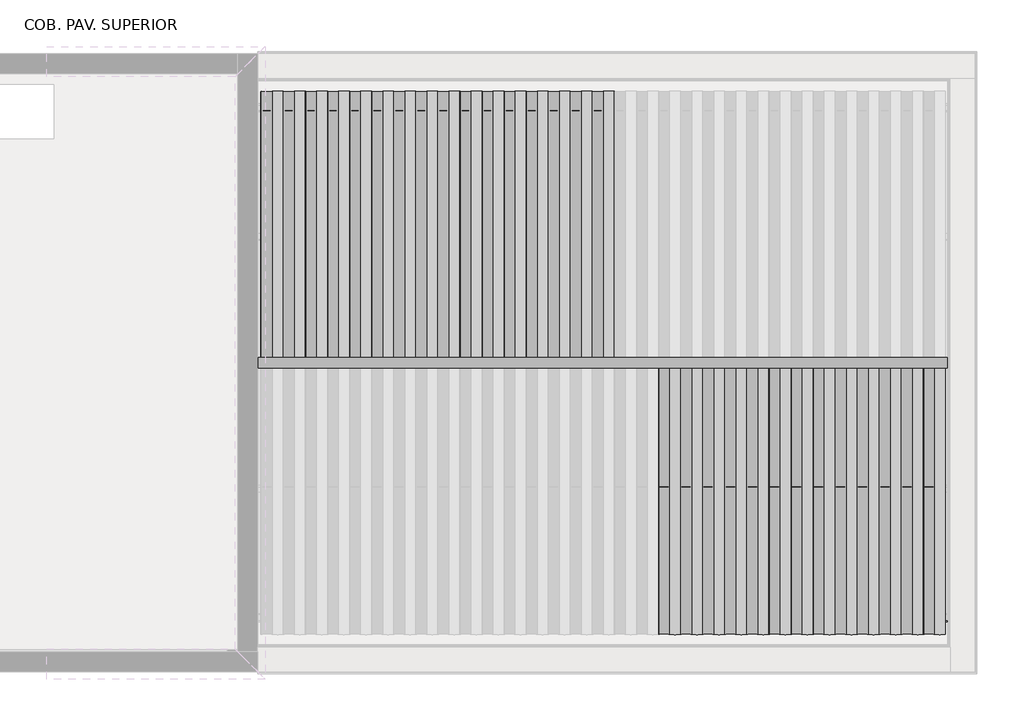
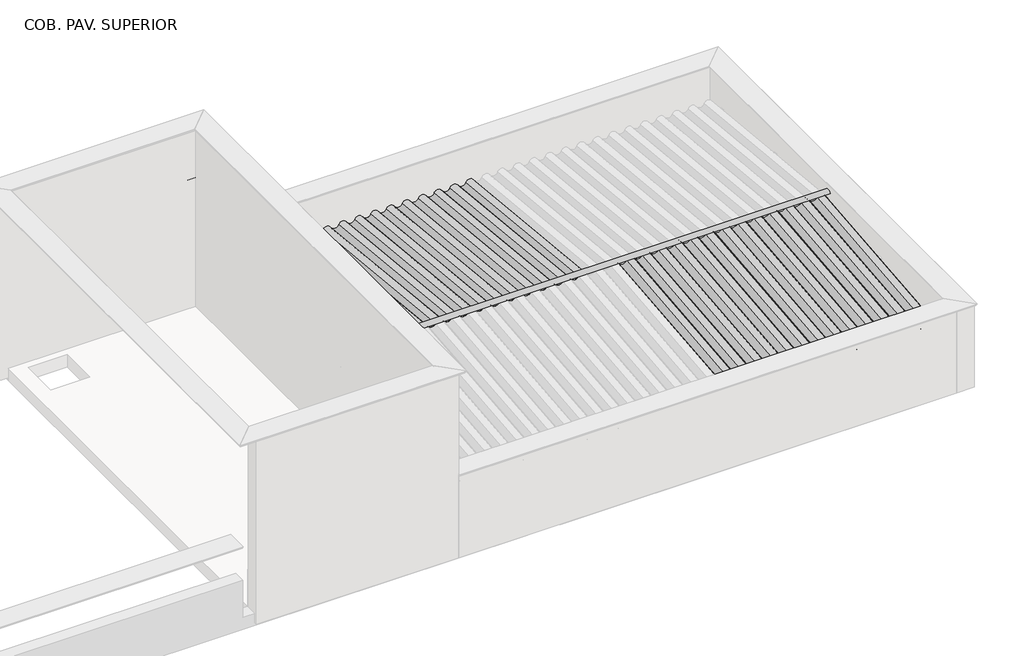
# One storey, part 6 of 7: 39 beams, 8 columns.
"""IFC4 building model written with IfcOpenShell, lengths in millimetres."""

import ifcopenshell
import ifcopenshell.guid

model = None  # the IFC model being written
_history = None  # IfcOwnerHistory: only IFC2X3 demands one
_inside = {}  # id of a spatial element -> (the spatial element, [elements in it])
_under = {}  # id of a project, library or spatial element -> (it, [spatial elements below it])
_declared = {}  # id of a project -> (the project, [libraries it declares])
_typed = {}  # id of a type object -> (the type object, [elements of that type])
_made_of = {}  # id of a material, layer set ... -> (it, [elements and type objects made of it])


def new_model(schema):
    """Start an empty IFC model of exactly this schema.

    Asked for "IFC4X3", IfcOpenShell would pick the latest addendum, in which some entities
    have other attributes; the version numbers below select the first issue.
    IFC2X3 requires an IfcOwnerHistory on every rooted entity: one is made here for all.
    """
    global model, _history
    if schema == "IFC4X3":
        model = ifcopenshell.file(schema_version=(4, 3, 0, 0))
    else:
        model = ifcopenshell.file(schema=schema)
    _inside.clear()
    _under.clear()
    _declared.clear()
    _typed.clear()
    _made_of.clear()
    _history = None
    if model.schema == "IFC2X3":
        org = make("IfcOrganization", Name="unknown")
        user = make(
            "IfcPersonAndOrganization",
            ThePerson=make("IfcPerson", FamilyName="unknown"),
            TheOrganization=org,
        )
        app = make(
            "IfcApplication",
            ApplicationDeveloper=org,
            Version="unknown",
            ApplicationFullName="unknown",
            ApplicationIdentifier="unknown",
        )
        _history = make(
            "IfcOwnerHistory",
            OwningUser=user,
            OwningApplication=app,
            ChangeAction="ADDED",
            CreationDate=0,
        )
    return model


def make(cls, **values):
    """One entity of the class cls with the attributes given. An attribute that is None is left unset."""
    return model.create_entity(
        cls, **{name: value for name, value in values.items() if value is not None}
    )


def rooted(cls, **values):
    """An entity with a GlobalId (a new one), such as an element, a storey or a relation."""
    return make(cls, GlobalId=ifcopenshell.guid.new(), OwnerHistory=_history, **values)


def si_unit(unit_type, name, prefix=None):
    """IfcSIUnit, for example si_unit("LENGTHUNIT", "METRE", prefix="MILLI")."""
    return make("IfcSIUnit", UnitType=unit_type, Prefix=prefix, Name=name)


def assignment(units):
    """IfcUnitAssignment: the units of a project."""
    return None if units is None else make("IfcUnitAssignment", Units=units)


def point(xyz):
    """IfcCartesianPoint."""
    return None if xyz is None else make("IfcCartesianPoint", Coordinates=xyz)


def direction(xyz):
    """IfcDirection."""
    return None if xyz is None else make("IfcDirection", DirectionRatios=xyz)


def frame(location, z_axis=None, x_axis=None):
    """IfcAxis2Placement3D, a coordinate frame: its origin and axes. An axis left out is left unset."""
    return make(
        "IfcAxis2Placement3D",
        Location=point(location),
        Axis=direction(z_axis),
        RefDirection=direction(x_axis),
    )


def frame_2d(location, x_axis=None):
    """IfcAxis2Placement2D, a coordinate frame in the plane: its origin and x axis."""
    return make(
        "IfcAxis2Placement2D", Location=point(location), RefDirection=direction(x_axis)
    )


def origin():
    """The frame at (0, 0, 0) with its axes left unset."""
    return frame((0.0, 0.0, 0.0))


def place(relative_to, where):
    """IfcLocalPlacement: puts the frame where relative to a parent placement (None: the world)."""
    return make(
        "IfcLocalPlacement", PlacementRelTo=relative_to, RelativePlacement=where
    )


def context(
    kind, dimensions, precision=None, world=None, true_north=None, identifier=None
):
    """IfcGeometricRepresentationContext, for example the 3D "Model" context."""
    return make(
        "IfcGeometricRepresentationContext",
        ContextIdentifier=identifier,
        ContextType=kind,
        CoordinateSpaceDimension=dimensions,
        Precision=precision,
        WorldCoordinateSystem=world,
        TrueNorth=true_north,
    )


def project(units=None, contexts=None):
    """IfcProject with its units and contexts."""
    return rooted(
        "IfcProject",
        Name="project",
        RepresentationContexts=contexts,
        UnitsInContext=assignment(units),
    )


def spatial(cls, under=None, at=None, **own):
    """A site, building, storey or space (cls), placed at a placement, below another one or the project."""
    s = rooted(cls, ObjectPlacement=at, **own)
    if under is not None:
        _under.setdefault(under.id(), (under, []))[1].append(s)
    return s


def polyline(points):
    """IfcPolyline through the points."""
    return make("IfcPolyline", Points=[point(p) for p in points])


def circle_curve(where, radius):
    """IfcCircle in the frame where."""
    return make("IfcCircle", Position=where, Radius=radius)


def trimmed(basis, trim1, trim2, sense, master):
    """IfcTrimmedCurve: the piece of a basis curve between two trims."""
    return make(
        "IfcTrimmedCurve",
        BasisCurve=basis,
        Trim1=trim1,
        Trim2=trim2,
        SenseAgreement=sense,
        MasterRepresentation=master,
    )


def segment(curve, same_sense, transition):
    """IfcCompositeCurveSegment."""
    return make(
        "IfcCompositeCurveSegment",
        Transition=transition,
        SameSense=same_sense,
        ParentCurve=curve,
    )


def composite_curve(segments, self_intersect=None):
    """IfcCompositeCurve: segments joined end to end."""
    return make("IfcCompositeCurve", Segments=segments, SelfIntersect=self_intersect)


def outline(outer, holes=None, kind="AREA"):
    """IfcArbitraryClosedProfileDef: a profile drawn as a closed curve; with holes, ...WithVoids."""
    if holes is None:
        return make("IfcArbitraryClosedProfileDef", ProfileType=kind, OuterCurve=outer)
    return make(
        "IfcArbitraryProfileDefWithVoids",
        ProfileType=kind,
        OuterCurve=outer,
        InnerCurves=holes,
    )


def extrude(swept, where, along, depth):
    """IfcExtrudedAreaSolid: the profile swept, set in the frame where, extruded along a direction by depth."""
    return make(
        "IfcExtrudedAreaSolid",
        SweptArea=swept,
        Position=where,
        ExtrudedDirection=direction(along),
        Depth=depth,
    )


def faces_of(points, faces, orient=None, outer=None):
    """IfcFace entities. A face is a list of loops; a loop is a list of indices into points, from 0.

    orient and outer hold one flag for each loop. By default every Orientation is true, the
    first loop of a face is its IfcFaceOuterBound and the others are IfcFaceBound.
    """
    made = []
    for i, loops in enumerate(faces):
        bounds = []
        for j, loop in enumerate(loops):
            is_outer = j == 0 if outer is None else outer[i][j]
            bounds.append(
                make(
                    "IfcFaceOuterBound" if is_outer else "IfcFaceBound",
                    Bound=make("IfcPolyLoop", Polygon=[points[k] for k in loop]),
                    Orientation=True if orient is None else orient[i][j],
                )
            )
        made.append(make("IfcFace", Bounds=bounds))
    return made


def faceted_brep(points, faces, orient=None, outer=None, voids=None):
    """IfcFacetedBrep: a solid bounded by flat faces; with voids (closed shells), ...WithVoids."""
    shared = [point(p) for p in points]
    hull = make("IfcClosedShell", CfsFaces=faces_of(shared, faces, orient, outer))
    if voids is None:
        return make("IfcFacetedBrep", Outer=hull)
    return make(
        "IfcFacetedBrepWithVoids",
        Outer=hull,
        Voids=[
            make(cls, CfsFaces=faces_of(shared, fs, o, b)) for cls, fs, o, b in voids
        ],
    )


def shape(context_of_items, identifier, shape_type, items):
    """IfcShapeRepresentation: the items that make up one representation, for example the "Body"."""
    return make(
        "IfcShapeRepresentation",
        ContextOfItems=context_of_items,
        RepresentationIdentifier=identifier,
        RepresentationType=shape_type,
        Items=items,
    )


def source(mapping_origin, context_of_items, identifier, shape_type, items):
    """IfcRepresentationMap: a shape defined once, which mapped items show again and again."""
    return make(
        "IfcRepresentationMap",
        MappingOrigin=mapping_origin,
        MappedRepresentation=shape(context_of_items, identifier, shape_type, items),
    )


def transform(
    local_origin,
    x_axis=None,
    y_axis=None,
    z_axis=None,
    scale=None,
    scale2=None,
    scale3=None,
    uniform=True,
):
    """IfcCartesianTransformationOperator3D, or its non-uniform kind. x_axis, y_axis, z_axis: its Axis1, 2, 3."""
    if uniform:
        return make(
            "IfcCartesianTransformationOperator3D",
            Axis1=direction(x_axis),
            Axis2=direction(y_axis),
            LocalOrigin=point(local_origin),
            Scale=scale,
            Axis3=direction(z_axis),
        )
    return make(
        "IfcCartesianTransformationOperator3DnonUniform",
        Axis1=direction(x_axis),
        Axis2=direction(y_axis),
        LocalOrigin=point(local_origin),
        Scale=scale,
        Axis3=direction(z_axis),
        Scale2=scale2,
        Scale3=scale3,
    )


def mapped(mapping_source, mapping_target):
    """IfcMappedItem: shows the shape of a source again, moved by a transform."""
    return make(
        "IfcMappedItem", MappingSource=mapping_source, MappingTarget=mapping_target
    )


def made_of(thing, what):
    """Note that an element or type object is made of a material, layer set ...; save() writes the relation."""
    if what is not None:
        _made_of.setdefault(what.id(), (what, []))[1].append(thing)
    return thing


def element(
    cls,
    number,
    at=None,
    inside=None,
    cuts=None,
    type_object=None,
    material=None,
    context=None,
    identifier="Body",
    shape_type=None,
    held_by="IfcProductDefinitionShape",
    body=None,
    shapes=None,
    **own,
):
    """One element of the class cls, such as IfcWall. Its Tag is "e" and its number.

    at: its placement. inside: the storey or other place that contains it. cuts: it is an
    opening in that element (IfcRelVoidsElement). A single representation is given by context,
    identifier, shape_type and body (its items); several are given by shapes. held_by: the class
    of the entity that holds the representations. save() writes the other relations.
    """
    e = rooted(cls, Tag="e%d" % number, ObjectPlacement=at, **own)
    if body is not None:
        shapes = [shape(context, identifier, shape_type, body)]
    if shapes is not None:
        e.Representation = make(held_by, Representations=shapes)
    if inside is not None:
        _inside.setdefault(inside.id(), (inside, []))[1].append(e)
    if cuts is not None:
        rooted(
            "IfcRelVoidsElement", RelatingBuildingElement=cuts, RelatedOpeningElement=e
        )
    if type_object is not None:
        _typed.setdefault(type_object.id(), (type_object, []))[1].append(e)
    return made_of(e, material)


def aggregate(whole, parts):
    """IfcRelAggregates: a whole, such as a stair, and the parts it consists of."""
    return rooted("IfcRelAggregates", RelatingObject=whole, RelatedObjects=parts)


def save(model, path):
    """Write the relations noted so far, then the file.

    IfcRelAggregates (storeys below a building ...), IfcRelContainedInSpatialStructure (elements
    in a storey), IfcRelDefinesByType, IfcRelAssociatesMaterial and IfcRelDeclares: one each for
    every whole, place, type object, material and project.
    """
    for whole, parts in _under.values():
        aggregate(whole, parts)
    for where, things in _inside.values():
        rooted(
            "IfcRelContainedInSpatialStructure",
            RelatedElements=things,
            RelatingStructure=where,
        )
    for kind, things in _typed.values():
        rooted("IfcRelDefinesByType", RelatedObjects=things, RelatingType=kind)
    for what, things in _made_of.values():
        rooted("IfcRelAssociatesMaterial", RelatedObjects=things, RelatingMaterial=what)
    for by, libraries in _declared.values():
        rooted("IfcRelDeclares", RelatingContext=by, RelatedDefinitions=libraries)
    model.write(path)


def cumeeira_telha_ondulada_fibrocimento_a8dbf5af(model_context):
    return source(origin(), model_context, "Body", "SweptSolid", [
        extrude(outline(composite_curve([segment(polyline([(58.3970135, 42.4437972), (53.9055884, 40.2467307)]), True, "CONTINUOUS"), segment(trimmed(circle_curve(frame_2d((-1.6029865, 13.0936483)), 61.7939461), [point((53.9055884, 40.2467307))], [point((-57.1115615, 40.2467307))], True, "CARTESIAN"), True, "CONTINUOUS"), segment(polyline([(-57.1115615, 40.2467307), (-61.6029865, 42.4437972)]), True, "CONTINUOUS"), segment(trimmed(circle_curve(frame_2d((-1.6029865, 13.0936483)), 66.7939461), [point((-61.6029865, 42.4437972))], [point((58.3970135, 42.4437972))], False, "CARTESIAN"), True, "CONTINUOUS")], self_intersect=False)), frame((-3970.0, 0.0, 0.0), z_axis=(1.0, 0.0, 0.0), x_axis=(0.0, 1.0, 0.0)), (0.0, 0.0, 1.0), 7940.0),
    ])


def viga_cumeeira_6x16cm_8fcfcc43(model_context):
    return source(origin(), model_context, "Body", "SweptSolid", [
        extrude(outline(polyline([(3822.5, 30.0), (3822.5, -30.0), (-3822.5, -30.0), (-3822.5, 30.0), (3822.5, 30.0)])), frame((0.0, 0.0, -80.0), z_axis=(0.0, 0.0, 1.0), x_axis=(1.0, 0.0, 0.0)), (0.0, 0.0, 1.0), 160.0),
    ])


def column_d505325c(model_context):
    return source(origin(), model_context, "Body", "SweptSolid", [
        extrude(outline(polyline([(30.0, 80.0), (30.0, -80.0), (-30.0, -80.0), (-30.0, 80.0), (30.0, 80.0)])), frame((0.0, 0.0, 6710.0), z_axis=(0.0, 0.0, 1.0), x_axis=(1.0, 0.0, 0.0)), (0.0, 0.0, 1.0), 750.0),
    ])


def column_4db371bd(model_context):
    return source(origin(), model_context, "Body", "SweptSolid", [
        extrude(outline(polyline([(30.0, 80.0), (30.0, -80.0), (-30.0, -80.0), (-30.0, 80.0), (30.0, 80.0)])), frame((0.0, 0.0, 6710.0), z_axis=(0.0, 0.0, 1.0), x_axis=(1.0, 0.0, 0.0)), (0.0, 0.0, 1.0), 660.0),
    ])


def column_e8b88e91(model_context):
    return source(origin(), model_context, "Body", "SweptSolid", [
        extrude(outline(polyline([(30.0, 80.0), (30.0, -80.0), (-30.0, -80.0), (-30.0, 80.0), (30.0, 80.0)])), frame((0.0, 0.0, 6710.0), z_axis=(0.0, 0.0, 1.0), x_axis=(1.0, 0.0, 0.0)), (0.0, 0.0, 1.0), 515.0),
    ])


model = new_model("IFC4")

# Units and contexts
model_context = context("Model", 3, world=origin())
ifc_project = project(units=[si_unit("LENGTHUNIT", "METRE", prefix="MILLI")], contexts=[model_context])

# Site, building, storey
site = spatial("IfcSite", under=ifc_project)
building = spatial("IfcBuilding", under=site)
storey = spatial("IfcBuildingStorey", under=building, Name="COB. PAV. SUPERIOR", Elevation=6650.0)

# Beams
placement = place(None, origin())
element("IfcBeam", 1, at=placement, inside=storey, context=model_context, shape_type="SweptSolid", body=[
    extrude(outline(polyline([(5090.718693, -7711.5607799), (5090.718693, -7831.5607799), (3090.718693, -7831.5607799), (3090.718693, -7711.5607799), (5090.718693, -7711.5607799)])), frame((0.0, 0.0, 6650.0), z_axis=(0.0, 0.0, 1.0), x_axis=(1.0, 0.0, 0.0)), (0.0, 0.0, 1.0), 60.0),
])
element("IfcBeam", 2, at=placement, inside=storey, context=model_context, shape_type="SweptSolid", body=[
    extrude(outline(polyline([(7090.718693, -7711.5607799), (7090.718693, -7831.5607799), (5090.718693, -7831.5607799), (5090.718693, -7711.5607799), (7090.718693, -7711.5607799)])), frame((0.0, 0.0, 6650.0), z_axis=(0.0, 0.0, 1.0), x_axis=(1.0, 0.0, 0.0)), (0.0, 0.0, 1.0), 60.0),
])
element("IfcBeam", 3, at=placement, inside=storey, context=model_context, shape_type="SweptSolid", body=[
    extrude(outline(polyline([(5089.7186924, -6319.8711004), (5089.7186924, -6439.8711004), (3089.718693, -6439.8711004), (3089.718693, -6319.8711004), (5089.7186924, -6319.8711004)])), frame((0.0, 0.0, 6650.0), z_axis=(0.0, 0.0, 1.0), x_axis=(1.0, 0.0, 0.0)), (0.0, 0.0, 1.0), 60.0),
])
element("IfcBeam", 4, at=placement, inside=storey, context=model_context, shape_type="SweptSolid", body=[
    extrude(outline(polyline([(7089.7186924, -6319.8711004), (7089.7186924, -6439.8711004), (5089.7186936, -6439.8711004), (5089.7186936, -6319.8711004), (7089.7186924, -6319.8711004)])), frame((0.0, 0.0, 6650.0), z_axis=(0.0, 0.0, 1.0), x_axis=(1.0, 0.0, 0.0)), (0.0, 0.0, 1.0), 60.0),
])
element("IfcBeam", 5, at=placement, inside=storey, context=model_context, shape_type="SweptSolid", body=[
    extrude(outline(polyline([(9089.718693, -9101.268869), (9089.718693, -9221.268869), (7089.718693, -9221.268869), (7089.718693, -9101.268869), (9089.718693, -9101.268869)])), frame((0.0, 0.0, 6650.0), z_axis=(0.0, 0.0, 1.0), x_axis=(1.0, 0.0, 0.0)), (0.0, 0.0, 1.0), 60.0),
])
element("IfcBeam", 6, at=placement, inside=storey, context=model_context, shape_type="SweptSolid", body=[
    extrude(outline(polyline([(9089.718693, -10521.818869), (9089.718693, -10641.818869), (7089.718693, -10641.818869), (7089.718693, -10521.818869), (9089.718693, -10521.818869)])), frame((0.0, 0.0, 6650.0), z_axis=(0.0, 0.0, 1.0), x_axis=(1.0, 0.0, 0.0)), (0.0, 0.0, 1.0), 60.0),
])
element("IfcBeam", 7, at=placement, inside=storey, context=model_context, shape_type="SweptSolid", body=[
    extrude(outline(polyline([(10709.718693, -9101.268869), (10709.718693, -9221.268869), (9089.718693, -9221.268869), (9089.718693, -9101.268869), (10709.718693, -9101.268869)])), frame((0.0, 0.0, 6650.0), z_axis=(0.0, 0.0, 1.0), x_axis=(1.0, 0.0, 0.0)), (0.0, 0.0, 1.0), 60.0),
])
element("IfcBeam", 8, at=placement, inside=storey, context=model_context, shape_type="SweptSolid", body=[
    extrude(outline(polyline([(10729.718693, -10521.818869), (10729.718693, -10641.818869), (9089.718693, -10641.818869), (9089.718693, -10521.818869), (10729.718693, -10521.818869)])), frame((0.0, 0.0, 6650.0), z_axis=(0.0, 0.0, 1.0), x_axis=(1.0, 0.0, 0.0)), (0.0, 0.0, 1.0), 60.0),
])
cumeeira_telha_ondulada_fibrocimento_shape = cumeeira_telha_ondulada_fibrocimento_a8dbf5af(model_context)
element("IfcBeam", 9, ObjectType="Cumeeira Telha Ondulada : Fibrocimento", at=placement, inside=storey, context=model_context, shape_type="MappedRepresentation", body=[
    mapped(cumeeira_telha_ondulada_fibrocimento_shape, transform((7061.718693, -7771.5607799, 7660.6251229), x_axis=(-1.0, 0.0, 0.0), y_axis=(0.0, -1.0, 0.0), z_axis=(0.0, 0.0, 1.0))),
])
element("IfcBeam", 10, ObjectType="Telha Ondulada : Fibrocimento", at=placement, inside=storey, context=model_context, shape_type="SweptSolid", body=[
    extrude(outline(composite_curve([segment(trimmed(circle_curve(frame_2d((-58.7002978, -53.2060539)), 66.7939461), [point((-29.3501489, 6.7939461))], [point((-29.3501489, -113.2060539))], False, "CARTESIAN"), True, "CONTINUOUS"), segment(polyline([(-29.3501489, -113.2060539), (-31.5472154, -108.7146289)]), True, "CONTINUOUS"), segment(trimmed(circle_curve(frame_2d((-58.7002978, -53.2060539)), 61.7939461), [point((-31.5472154, -108.7146289))], [point((-31.5472154, 2.3025211))], True, "CARTESIAN"), True, "CONTINUOUS"), segment(trimmed(circle_curve(frame_2d((0.0, 66.7939461)), 71.7939461), [point((-31.5472154, 2.3025211))], [point((-31.5472154, 131.2853711))], False, "CARTESIAN"), True, "CONTINUOUS"), segment(polyline([(-31.5472154, 131.2853711), (-29.3501489, 126.7939461)]), True, "CONTINUOUS"), segment(trimmed(circle_curve(frame_2d((0.0, 66.7939461)), 66.7939461), [point((-29.3501489, 126.7939461))], [point((-29.3501489, 6.7939461))], True, "CARTESIAN"), True, "CONTINUOUS")], self_intersect=False)), frame((3256.1156257, -4759.1621575, 7394.5315886), z_axis=(0.0, -0.9950371902099893, 0.09950371902099778), x_axis=(0.0, 0.09950371902099778, 0.9950371902099893)), (0.0, 0.0, 1.0), 3017.2387654),
])
element("IfcBeam", 11, ObjectType="Telha Ondulada : Fibrocimento", at=placement, inside=storey, context=model_context, shape_type="SweptSolid", body=[
    extrude(outline(composite_curve([segment(trimmed(circle_curve(frame_2d((-58.7002978, -53.2060539)), 66.7939461), [point((-29.3501489, 6.7939461))], [point((-29.3501489, -113.2060539))], False, "CARTESIAN"), True, "CONTINUOUS"), segment(polyline([(-29.3501489, -113.2060539), (-31.5472154, -108.7146289)]), True, "CONTINUOUS"), segment(trimmed(circle_curve(frame_2d((-58.7002978, -53.2060539)), 61.7939461), [point((-31.5472154, -108.7146289))], [point((-31.5472154, 2.3025211))], True, "CARTESIAN"), True, "CONTINUOUS"), segment(trimmed(circle_curve(frame_2d((0.0, 66.7939461)), 71.7939461), [point((-31.5472154, 2.3025211))], [point((-31.5472154, 131.2853711))], False, "CARTESIAN"), True, "CONTINUOUS"), segment(polyline([(-31.5472154, 131.2853711), (-29.3501489, 126.7939461)]), True, "CONTINUOUS"), segment(trimmed(circle_curve(frame_2d((0.0, 66.7939461)), 66.7939461), [point((-29.3501489, 126.7939461))], [point((-29.3501489, 6.7939461))], True, "CARTESIAN"), True, "CONTINUOUS")], self_intersect=False)), frame((3500.6156257, -4759.1621575, 7394.5315886), z_axis=(0.0, -0.9950371902099893, 0.09950371902099778), x_axis=(0.0, 0.09950371902099778, 0.9950371902099893)), (0.0, 0.0, 1.0), 3017.2387654),
])
element("IfcBeam", 12, ObjectType="Telha Ondulada : Fibrocimento", at=placement, inside=storey, context=model_context, shape_type="SweptSolid", body=[
    extrude(outline(composite_curve([segment(trimmed(circle_curve(frame_2d((-58.7002978, -53.2060539)), 66.7939461), [point((-29.3501489, 6.7939461))], [point((-29.3501489, -113.2060539))], False, "CARTESIAN"), True, "CONTINUOUS"), segment(polyline([(-29.3501489, -113.2060539), (-31.5472154, -108.7146289)]), True, "CONTINUOUS"), segment(trimmed(circle_curve(frame_2d((-58.7002978, -53.2060539)), 61.7939461), [point((-31.5472154, -108.7146289))], [point((-31.5472154, 2.3025211))], True, "CARTESIAN"), True, "CONTINUOUS"), segment(trimmed(circle_curve(frame_2d((0.0, 66.7939461)), 71.7939461), [point((-31.5472154, 2.3025211))], [point((-31.5472154, 131.2853711))], False, "CARTESIAN"), True, "CONTINUOUS"), segment(polyline([(-31.5472154, 131.2853711), (-29.3501489, 126.7939461)]), True, "CONTINUOUS"), segment(trimmed(circle_curve(frame_2d((0.0, 66.7939461)), 66.7939461), [point((-29.3501489, 126.7939461))], [point((-29.3501489, 6.7939461))], True, "CARTESIAN"), True, "CONTINUOUS")], self_intersect=False)), frame((3745.1156257, -4759.1621575, 7394.5315886), z_axis=(0.0, -0.9950371902099893, 0.09950371902099776), x_axis=(0.0, 0.09950371902099776, 0.9950371902099893)), (0.0, 0.0, 1.0), 3017.2387654),
])
element("IfcBeam", 13, ObjectType="Telha Ondulada : Fibrocimento", at=placement, inside=storey, context=model_context, shape_type="SweptSolid", body=[
    extrude(outline(composite_curve([segment(trimmed(circle_curve(frame_2d((-58.7002978, -53.2060539)), 66.7939461), [point((-29.3501489, 6.7939461))], [point((-29.3501489, -113.2060539))], False, "CARTESIAN"), True, "CONTINUOUS"), segment(polyline([(-29.3501489, -113.2060539), (-31.5472154, -108.7146289)]), True, "CONTINUOUS"), segment(trimmed(circle_curve(frame_2d((-58.7002978, -53.2060539)), 61.7939461), [point((-31.5472154, -108.7146289))], [point((-31.5472154, 2.3025211))], True, "CARTESIAN"), True, "CONTINUOUS"), segment(trimmed(circle_curve(frame_2d((0.0, 66.7939461)), 71.7939461), [point((-31.5472154, 2.3025211))], [point((-31.5472154, 131.2853711))], False, "CARTESIAN"), True, "CONTINUOUS"), segment(polyline([(-31.5472154, 131.2853711), (-29.3501489, 126.7939461)]), True, "CONTINUOUS"), segment(trimmed(circle_curve(frame_2d((0.0, 66.7939461)), 66.7939461), [point((-29.3501489, 126.7939461))], [point((-29.3501489, 6.7939461))], True, "CARTESIAN"), True, "CONTINUOUS")], self_intersect=False)), frame((3989.6156257, -4759.1621575, 7394.5315886), z_axis=(0.0, -0.9950371902099893, 0.09950371902099776), x_axis=(0.0, 0.09950371902099776, 0.9950371902099893)), (0.0, 0.0, 1.0), 3017.2387654),
])
element("IfcBeam", 14, ObjectType="Telha Ondulada : Fibrocimento", at=placement, inside=storey, context=model_context, shape_type="SweptSolid", body=[
    extrude(outline(composite_curve([segment(trimmed(circle_curve(frame_2d((-58.7002978, -53.2060539)), 66.7939461), [point((-29.3501489, 6.7939461))], [point((-29.3501489, -113.2060539))], False, "CARTESIAN"), True, "CONTINUOUS"), segment(polyline([(-29.3501489, -113.2060539), (-31.5472154, -108.7146289)]), True, "CONTINUOUS"), segment(trimmed(circle_curve(frame_2d((-58.7002978, -53.2060539)), 61.7939461), [point((-31.5472154, -108.7146289))], [point((-31.5472154, 2.3025211))], True, "CARTESIAN"), True, "CONTINUOUS"), segment(trimmed(circle_curve(frame_2d((0.0, 66.7939461)), 71.7939461), [point((-31.5472154, 2.3025211))], [point((-31.5472154, 131.2853711))], False, "CARTESIAN"), True, "CONTINUOUS"), segment(polyline([(-31.5472154, 131.2853711), (-29.3501489, 126.7939461)]), True, "CONTINUOUS"), segment(trimmed(circle_curve(frame_2d((0.0, 66.7939461)), 66.7939461), [point((-29.3501489, 126.7939461))], [point((-29.3501489, 6.7939461))], True, "CARTESIAN"), True, "CONTINUOUS")], self_intersect=False)), frame((4234.1156257, -4759.1621575, 7394.5315886), z_axis=(0.0, -0.9950371902099893, 0.09950371902099775), x_axis=(0.0, 0.09950371902099775, 0.9950371902099893)), (0.0, 0.0, 1.0), 3017.2387654),
])
element("IfcBeam", 15, ObjectType="Telha Ondulada : Fibrocimento", at=placement, inside=storey, context=model_context, shape_type="SweptSolid", body=[
    extrude(outline(composite_curve([segment(trimmed(circle_curve(frame_2d((-58.7002978, -53.2060539)), 66.7939461), [point((-29.3501489, 6.7939461))], [point((-29.3501489, -113.2060539))], False, "CARTESIAN"), True, "CONTINUOUS"), segment(polyline([(-29.3501489, -113.2060539), (-31.5472154, -108.7146289)]), True, "CONTINUOUS"), segment(trimmed(circle_curve(frame_2d((-58.7002978, -53.2060539)), 61.7939461), [point((-31.5472154, -108.7146289))], [point((-31.5472154, 2.3025211))], True, "CARTESIAN"), True, "CONTINUOUS"), segment(trimmed(circle_curve(frame_2d((0.0, 66.7939461)), 71.7939461), [point((-31.5472154, 2.3025211))], [point((-31.5472154, 131.2853711))], False, "CARTESIAN"), True, "CONTINUOUS"), segment(polyline([(-31.5472154, 131.2853711), (-29.3501489, 126.7939461)]), True, "CONTINUOUS"), segment(trimmed(circle_curve(frame_2d((0.0, 66.7939461)), 66.7939461), [point((-29.3501489, 126.7939461))], [point((-29.3501489, 6.7939461))], True, "CARTESIAN"), True, "CONTINUOUS")], self_intersect=False)), frame((4478.6156257, -4759.1621575, 7394.5315886), z_axis=(0.0, -0.9950371902099893, 0.09950371902099778), x_axis=(0.0, 0.09950371902099778, 0.9950371902099893)), (0.0, 0.0, 1.0), 3017.2387654),
])
element("IfcBeam", 16, ObjectType="Telha Ondulada : Fibrocimento", at=placement, inside=storey, context=model_context, shape_type="SweptSolid", body=[
    extrude(outline(composite_curve([segment(trimmed(circle_curve(frame_2d((-58.7002978, -53.2060539)), 66.7939461), [point((-29.3501489, 6.7939461))], [point((-29.3501489, -113.2060539))], False, "CARTESIAN"), True, "CONTINUOUS"), segment(polyline([(-29.3501489, -113.2060539), (-31.5472154, -108.7146289)]), True, "CONTINUOUS"), segment(trimmed(circle_curve(frame_2d((-58.7002978, -53.2060539)), 61.7939461), [point((-31.5472154, -108.7146289))], [point((-31.5472154, 2.3025211))], True, "CARTESIAN"), True, "CONTINUOUS"), segment(trimmed(circle_curve(frame_2d((0.0, 66.7939461)), 71.7939461), [point((-31.5472154, 2.3025211))], [point((-31.5472154, 131.2853711))], False, "CARTESIAN"), True, "CONTINUOUS"), segment(polyline([(-31.5472154, 131.2853711), (-29.3501489, 126.7939461)]), True, "CONTINUOUS"), segment(trimmed(circle_curve(frame_2d((0.0, 66.7939461)), 66.7939461), [point((-29.3501489, 126.7939461))], [point((-29.3501489, 6.7939461))], True, "CARTESIAN"), True, "CONTINUOUS")], self_intersect=False)), frame((4723.1156257, -4759.1621575, 7394.5315886), z_axis=(0.0, -0.9950371902099893, 0.09950371902099776), x_axis=(0.0, 0.09950371902099776, 0.9950371902099893)), (0.0, 0.0, 1.0), 3017.2387654),
])
element("IfcBeam", 17, ObjectType="Telha Ondulada : Fibrocimento", at=placement, inside=storey, context=model_context, shape_type="SweptSolid", body=[
    extrude(outline(composite_curve([segment(trimmed(circle_curve(frame_2d((-58.7002978, -53.2060539)), 66.7939461), [point((-29.3501489, 6.7939461))], [point((-29.3501489, -113.2060539))], False, "CARTESIAN"), True, "CONTINUOUS"), segment(polyline([(-29.3501489, -113.2060539), (-31.5472154, -108.7146289)]), True, "CONTINUOUS"), segment(trimmed(circle_curve(frame_2d((-58.7002978, -53.2060539)), 61.7939461), [point((-31.5472154, -108.7146289))], [point((-31.5472154, 2.3025211))], True, "CARTESIAN"), True, "CONTINUOUS"), segment(trimmed(circle_curve(frame_2d((0.0, 66.7939461)), 71.7939461), [point((-31.5472154, 2.3025211))], [point((-31.5472154, 131.2853711))], False, "CARTESIAN"), True, "CONTINUOUS"), segment(polyline([(-31.5472154, 131.2853711), (-29.3501489, 126.7939461)]), True, "CONTINUOUS"), segment(trimmed(circle_curve(frame_2d((0.0, 66.7939461)), 66.7939461), [point((-29.3501489, 126.7939461))], [point((-29.3501489, 6.7939461))], True, "CARTESIAN"), True, "CONTINUOUS")], self_intersect=False)), frame((4967.6156257, -4759.1621575, 7394.5315886), z_axis=(0.0, -0.9950371902099893, 0.09950371902099775), x_axis=(0.0, 0.09950371902099775, 0.9950371902099893)), (0.0, 0.0, 1.0), 3017.2387654),
])
element("IfcBeam", 18, ObjectType="Telha Ondulada : Fibrocimento", at=placement, inside=storey, context=model_context, shape_type="SweptSolid", body=[
    extrude(outline(composite_curve([segment(trimmed(circle_curve(frame_2d((-58.7002978, -53.2060539)), 66.7939461), [point((-29.3501489, 6.7939461))], [point((-29.3501489, -113.2060539))], False, "CARTESIAN"), True, "CONTINUOUS"), segment(polyline([(-29.3501489, -113.2060539), (-31.5472154, -108.7146289)]), True, "CONTINUOUS"), segment(trimmed(circle_curve(frame_2d((-58.7002978, -53.2060539)), 61.7939461), [point((-31.5472154, -108.7146289))], [point((-31.5472154, 2.3025211))], True, "CARTESIAN"), True, "CONTINUOUS"), segment(trimmed(circle_curve(frame_2d((0.0, 66.7939461)), 71.7939461), [point((-31.5472154, 2.3025211))], [point((-31.5472154, 131.2853711))], False, "CARTESIAN"), True, "CONTINUOUS"), segment(polyline([(-31.5472154, 131.2853711), (-29.3501489, 126.7939461)]), True, "CONTINUOUS"), segment(trimmed(circle_curve(frame_2d((0.0, 66.7939461)), 66.7939461), [point((-29.3501489, 126.7939461))], [point((-29.3501489, 6.7939461))], True, "CARTESIAN"), True, "CONTINUOUS")], self_intersect=False)), frame((5212.1156257, -4759.1621575, 7394.5315886), z_axis=(0.0, -0.9950371902099893, 0.09950371902099778), x_axis=(0.0, 0.09950371902099778, 0.9950371902099893)), (0.0, 0.0, 1.0), 3017.2387654),
])
element("IfcBeam", 19, ObjectType="Telha Ondulada : Fibrocimento", at=placement, inside=storey, context=model_context, shape_type="SweptSolid", body=[
    extrude(outline(composite_curve([segment(trimmed(circle_curve(frame_2d((-58.7002978, -53.2060539)), 66.7939461), [point((-29.3501489, 6.7939461))], [point((-29.3501489, -113.2060539))], False, "CARTESIAN"), True, "CONTINUOUS"), segment(polyline([(-29.3501489, -113.2060539), (-31.5472154, -108.7146289)]), True, "CONTINUOUS"), segment(trimmed(circle_curve(frame_2d((-58.7002978, -53.2060539)), 61.7939461), [point((-31.5472154, -108.7146289))], [point((-31.5472154, 2.3025211))], True, "CARTESIAN"), True, "CONTINUOUS"), segment(trimmed(circle_curve(frame_2d((0.0, 66.7939461)), 71.7939461), [point((-31.5472154, 2.3025211))], [point((-31.5472154, 131.2853711))], False, "CARTESIAN"), True, "CONTINUOUS"), segment(polyline([(-31.5472154, 131.2853711), (-29.3501489, 126.7939461)]), True, "CONTINUOUS"), segment(trimmed(circle_curve(frame_2d((0.0, 66.7939461)), 66.7939461), [point((-29.3501489, 126.7939461))], [point((-29.3501489, 6.7939461))], True, "CARTESIAN"), True, "CONTINUOUS")], self_intersect=False)), frame((5456.6156257, -4759.1621575, 7394.5315886), z_axis=(0.0, -0.9950371902099893, 0.09950371902099776), x_axis=(0.0, 0.09950371902099776, 0.9950371902099893)), (0.0, 0.0, 1.0), 3017.2387654),
])
element("IfcBeam", 20, ObjectType="Telha Ondulada : Fibrocimento", at=placement, inside=storey, context=model_context, shape_type="SweptSolid", body=[
    extrude(outline(composite_curve([segment(trimmed(circle_curve(frame_2d((-58.7002978, -53.2060539)), 66.7939461), [point((-29.3501489, 6.7939461))], [point((-29.3501489, -113.2060539))], False, "CARTESIAN"), True, "CONTINUOUS"), segment(polyline([(-29.3501489, -113.2060539), (-31.5472154, -108.7146289)]), True, "CONTINUOUS"), segment(trimmed(circle_curve(frame_2d((-58.7002978, -53.2060539)), 61.7939461), [point((-31.5472154, -108.7146289))], [point((-31.5472154, 2.3025211))], True, "CARTESIAN"), True, "CONTINUOUS"), segment(trimmed(circle_curve(frame_2d((0.0, 66.7939461)), 71.7939461), [point((-31.5472154, 2.3025211))], [point((-31.5472154, 131.2853711))], False, "CARTESIAN"), True, "CONTINUOUS"), segment(polyline([(-31.5472154, 131.2853711), (-29.3501489, 126.7939461)]), True, "CONTINUOUS"), segment(trimmed(circle_curve(frame_2d((0.0, 66.7939461)), 66.7939461), [point((-29.3501489, 126.7939461))], [point((-29.3501489, 6.7939461))], True, "CARTESIAN"), True, "CONTINUOUS")], self_intersect=False)), frame((5701.1156257, -4759.1621575, 7394.5315886), z_axis=(0.0, -0.9950371902099893, 0.09950371902099776), x_axis=(0.0, 0.09950371902099776, 0.9950371902099893)), (0.0, 0.0, 1.0), 3017.2387654),
])
element("IfcBeam", 21, ObjectType="Telha Ondulada : Fibrocimento", at=placement, inside=storey, context=model_context, shape_type="SweptSolid", body=[
    extrude(outline(composite_curve([segment(trimmed(circle_curve(frame_2d((-58.7002978, -53.2060539)), 66.7939461), [point((-29.3501489, 6.7939461))], [point((-29.3501489, -113.2060539))], False, "CARTESIAN"), True, "CONTINUOUS"), segment(polyline([(-29.3501489, -113.2060539), (-31.5472154, -108.7146289)]), True, "CONTINUOUS"), segment(trimmed(circle_curve(frame_2d((-58.7002978, -53.2060539)), 61.7939461), [point((-31.5472154, -108.7146289))], [point((-31.5472154, 2.3025211))], True, "CARTESIAN"), True, "CONTINUOUS"), segment(trimmed(circle_curve(frame_2d((0.0, 66.7939461)), 71.7939461), [point((-31.5472154, 2.3025211))], [point((-31.5472154, 131.2853711))], False, "CARTESIAN"), True, "CONTINUOUS"), segment(polyline([(-31.5472154, 131.2853711), (-29.3501489, 126.7939461)]), True, "CONTINUOUS"), segment(trimmed(circle_curve(frame_2d((0.0, 66.7939461)), 66.7939461), [point((-29.3501489, 126.7939461))], [point((-29.3501489, 6.7939461))], True, "CARTESIAN"), True, "CONTINUOUS")], self_intersect=False)), frame((5945.6156257, -4759.1621575, 7394.5315886), z_axis=(0.0, -0.9950371902099893, 0.09950371902099778), x_axis=(0.0, 0.09950371902099778, 0.9950371902099893)), (0.0, 0.0, 1.0), 3017.2387654),
])
element("IfcBeam", 22, ObjectType="Telha Ondulada : Fibrocimento", at=placement, inside=storey, context=model_context, shape_type="SweptSolid", body=[
    extrude(outline(composite_curve([segment(trimmed(circle_curve(frame_2d((-58.7002978, -53.2060539)), 66.7939461), [point((-29.3501489, 6.7939461))], [point((-29.3501489, -113.2060539))], False, "CARTESIAN"), True, "CONTINUOUS"), segment(polyline([(-29.3501489, -113.2060539), (-31.5472154, -108.7146289)]), True, "CONTINUOUS"), segment(trimmed(circle_curve(frame_2d((-58.7002978, -53.2060539)), 61.7939461), [point((-31.5472154, -108.7146289))], [point((-31.5472154, 2.3025211))], True, "CARTESIAN"), True, "CONTINUOUS"), segment(trimmed(circle_curve(frame_2d((0.0, 66.7939461)), 71.7939461), [point((-31.5472154, 2.3025211))], [point((-31.5472154, 131.2853711))], False, "CARTESIAN"), True, "CONTINUOUS"), segment(polyline([(-31.5472154, 131.2853711), (-29.3501489, 126.7939461)]), True, "CONTINUOUS"), segment(trimmed(circle_curve(frame_2d((0.0, 66.7939461)), 66.7939461), [point((-29.3501489, 126.7939461))], [point((-29.3501489, 6.7939461))], True, "CARTESIAN"), True, "CONTINUOUS")], self_intersect=False)), frame((6190.1156257, -4759.1621575, 7394.5315886), z_axis=(0.0, -0.9950371902099893, 0.09950371902099778), x_axis=(0.0, 0.09950371902099778, 0.9950371902099893)), (0.0, 0.0, 1.0), 3017.2387654),
])
element("IfcBeam", 23, ObjectType="Telha Ondulada : Fibrocimento", at=placement, inside=storey, context=model_context, shape_type="SweptSolid", body=[
    extrude(outline(composite_curve([segment(trimmed(circle_curve(frame_2d((-58.7002978, -53.2060539)), 66.7939461), [point((-29.3501489, 6.7939461))], [point((-29.3501489, -113.2060539))], False, "CARTESIAN"), True, "CONTINUOUS"), segment(polyline([(-29.3501489, -113.2060539), (-31.5472154, -108.7146289)]), True, "CONTINUOUS"), segment(trimmed(circle_curve(frame_2d((-58.7002978, -53.2060539)), 61.7939461), [point((-31.5472154, -108.7146289))], [point((-31.5472154, 2.3025211))], True, "CARTESIAN"), True, "CONTINUOUS"), segment(trimmed(circle_curve(frame_2d((0.0, 66.7939461)), 71.7939461), [point((-31.5472154, 2.3025211))], [point((-31.5472154, 131.2853711))], False, "CARTESIAN"), True, "CONTINUOUS"), segment(polyline([(-31.5472154, 131.2853711), (-29.3501489, 126.7939461)]), True, "CONTINUOUS"), segment(trimmed(circle_curve(frame_2d((0.0, 66.7939461)), 66.7939461), [point((-29.3501489, 126.7939461))], [point((-29.3501489, 6.7939461))], True, "CARTESIAN"), True, "CONTINUOUS")], self_intersect=False)), frame((6434.6156257, -4759.1621575, 7394.5315886), z_axis=(0.0, -0.9950371902099893, 0.09950371902099776), x_axis=(0.0, 0.09950371902099776, 0.9950371902099893)), (0.0, 0.0, 1.0), 3017.2387654),
])
element("IfcBeam", 24, ObjectType="Telha Ondulada : Fibrocimento", at=placement, inside=storey, context=model_context, shape_type="SweptSolid", body=[
    extrude(outline(composite_curve([segment(trimmed(circle_curve(frame_2d((-58.7002978, -53.2060539)), 66.7939461), [point((-29.3501489, 6.7939461))], [point((-29.3501489, -113.2060539))], False, "CARTESIAN"), True, "CONTINUOUS"), segment(polyline([(-29.3501489, -113.2060539), (-31.5472154, -108.7146289)]), True, "CONTINUOUS"), segment(trimmed(circle_curve(frame_2d((-58.7002978, -53.2060539)), 61.7939461), [point((-31.5472154, -108.7146289))], [point((-31.5472154, 2.3025211))], True, "CARTESIAN"), True, "CONTINUOUS"), segment(trimmed(circle_curve(frame_2d((0.0, 66.7939461)), 71.7939461), [point((-31.5472154, 2.3025211))], [point((-31.5472154, 131.2853711))], False, "CARTESIAN"), True, "CONTINUOUS"), segment(polyline([(-31.5472154, 131.2853711), (-29.3501489, 126.7939461)]), True, "CONTINUOUS"), segment(trimmed(circle_curve(frame_2d((0.0, 66.7939461)), 66.7939461), [point((-29.3501489, 126.7939461))], [point((-29.3501489, 6.7939461))], True, "CARTESIAN"), True, "CONTINUOUS")], self_intersect=False)), frame((6679.1156257, -4759.1621575, 7394.5315886), z_axis=(0.0, -0.9950371902099893, 0.09950371902099776), x_axis=(0.0, 0.09950371902099776, 0.9950371902099893)), (0.0, 0.0, 1.0), 3017.2387654),
])
element("IfcBeam", 25, ObjectType="Telha Ondulada : Fibrocimento", at=placement, inside=storey, context=model_context, shape_type="SweptSolid", body=[
    extrude(outline(composite_curve([segment(trimmed(circle_curve(frame_2d((-58.7002978, -53.2060539)), 66.7939461), [point((-29.3501489, 6.7939461))], [point((-29.3501489, -113.2060539))], False, "CARTESIAN"), True, "CONTINUOUS"), segment(polyline([(-29.3501489, -113.2060539), (-31.5472154, -108.7146289)]), True, "CONTINUOUS"), segment(trimmed(circle_curve(frame_2d((-58.7002978, -53.2060539)), 61.7939461), [point((-31.5472154, -108.7146289))], [point((-31.5472154, 2.3025211))], True, "CARTESIAN"), True, "CONTINUOUS"), segment(trimmed(circle_curve(frame_2d((0.0, 66.7939461)), 71.7939461), [point((-31.5472154, 2.3025211))], [point((-31.5472154, 131.2853711))], False, "CARTESIAN"), True, "CONTINUOUS"), segment(polyline([(-31.5472154, 131.2853711), (-29.3501489, 126.7939461)]), True, "CONTINUOUS"), segment(trimmed(circle_curve(frame_2d((0.0, 66.7939461)), 66.7939461), [point((-29.3501489, 126.7939461))], [point((-29.3501489, 6.7939461))], True, "CARTESIAN"), True, "CONTINUOUS")], self_intersect=False)), frame((6923.6156257, -4759.1621575, 7394.5315886), z_axis=(0.0, -0.9950371902099893, 0.09950371902099775), x_axis=(0.0, 0.09950371902099775, 0.9950371902099893)), (0.0, 0.0, 1.0), 3017.2387654),
])
element("IfcBeam", 26, ObjectType="Telha Ondulada : Fibrocimento", at=placement, inside=storey, context=model_context, shape_type="SweptSolid", body=[
    extrude(outline(composite_curve([segment(trimmed(circle_curve(frame_2d((0.0, 66.7939461)), 66.7939461), [point((29.3501489, 6.7939461))], [point((29.3501489, 126.7939461))], True, "CARTESIAN"), True, "CONTINUOUS"), segment(polyline([(29.3501489, 126.7939461), (31.5472154, 131.2853711)]), True, "CONTINUOUS"), segment(trimmed(circle_curve(frame_2d((0.0, 66.7939461)), 71.7939461), [point((31.5472154, 131.2853711))], [point((31.5472154, 2.3025211))], False, "CARTESIAN"), True, "CONTINUOUS"), segment(trimmed(circle_curve(frame_2d((58.7002978, -53.2060539)), 61.7939461), [point((31.5472154, 2.3025211))], [point((31.5472154, -108.7146289))], True, "CARTESIAN"), True, "CONTINUOUS"), segment(polyline([(31.5472154, -108.7146289), (29.3501489, -113.2060539)]), True, "CONTINUOUS"), segment(trimmed(circle_curve(frame_2d((58.7002978, -53.2060539)), 66.7939461), [point((29.3501489, -113.2060539))], [point((29.3501489, 6.7939461))], False, "CARTESIAN"), True, "CONTINUOUS")], self_intersect=False)), frame((7657.1156257, -10781.9594023, 7394.5315886), z_axis=(0.0, 0.9950371902099894, 0.09950371902099747), x_axis=(0.0, 0.09950371902099747, -0.9950371902099894)), (0.0, 0.0, 1.0), 3017.2387654),
])
element("IfcBeam", 27, ObjectType="Telha Ondulada : Fibrocimento", at=placement, inside=storey, context=model_context, shape_type="SweptSolid", body=[
    extrude(outline(composite_curve([segment(trimmed(circle_curve(frame_2d((0.0, 66.7939461)), 66.7939461), [point((29.3501489, 6.7939461))], [point((29.3501489, 126.7939461))], True, "CARTESIAN"), True, "CONTINUOUS"), segment(polyline([(29.3501489, 126.7939461), (31.5472154, 131.2853711)]), True, "CONTINUOUS"), segment(trimmed(circle_curve(frame_2d((0.0, 66.7939461)), 71.7939461), [point((31.5472154, 131.2853711))], [point((31.5472154, 2.3025211))], False, "CARTESIAN"), True, "CONTINUOUS"), segment(trimmed(circle_curve(frame_2d((58.7002978, -53.2060539)), 61.7939461), [point((31.5472154, 2.3025211))], [point((31.5472154, -108.7146289))], True, "CARTESIAN"), True, "CONTINUOUS"), segment(polyline([(31.5472154, -108.7146289), (29.3501489, -113.2060539)]), True, "CONTINUOUS"), segment(trimmed(circle_curve(frame_2d((58.7002978, -53.2060539)), 66.7939461), [point((29.3501489, -113.2060539))], [point((29.3501489, 6.7939461))], False, "CARTESIAN"), True, "CONTINUOUS")], self_intersect=False)), frame((7901.6156257, -10781.9594023, 7394.5315886), z_axis=(0.0, 0.9950371902099894, 0.09950371902099751), x_axis=(0.0, 0.09950371902099751, -0.9950371902099894)), (0.0, 0.0, 1.0), 3017.2387654),
])
element("IfcBeam", 28, ObjectType="Telha Ondulada : Fibrocimento", at=placement, inside=storey, context=model_context, shape_type="SweptSolid", body=[
    extrude(outline(composite_curve([segment(trimmed(circle_curve(frame_2d((0.0, 66.7939461)), 66.7939461), [point((29.3501489, 6.7939461))], [point((29.3501489, 126.7939461))], True, "CARTESIAN"), True, "CONTINUOUS"), segment(polyline([(29.3501489, 126.7939461), (31.5472154, 131.2853711)]), True, "CONTINUOUS"), segment(trimmed(circle_curve(frame_2d((0.0, 66.7939461)), 71.7939461), [point((31.5472154, 131.2853711))], [point((31.5472154, 2.3025211))], False, "CARTESIAN"), True, "CONTINUOUS"), segment(trimmed(circle_curve(frame_2d((58.7002978, -53.2060539)), 61.7939461), [point((31.5472154, 2.3025211))], [point((31.5472154, -108.7146289))], True, "CARTESIAN"), True, "CONTINUOUS"), segment(polyline([(31.5472154, -108.7146289), (29.3501489, -113.2060539)]), True, "CONTINUOUS"), segment(trimmed(circle_curve(frame_2d((58.7002978, -53.2060539)), 66.7939461), [point((29.3501489, -113.2060539))], [point((29.3501489, 6.7939461))], False, "CARTESIAN"), True, "CONTINUOUS")], self_intersect=False)), frame((8146.1156257, -10781.9594023, 7394.5315886), z_axis=(0.0, 0.9950371902099894, 0.09950371902099751), x_axis=(0.0, 0.09950371902099751, -0.9950371902099894)), (0.0, 0.0, 1.0), 3017.2387654),
])
element("IfcBeam", 29, ObjectType="Telha Ondulada : Fibrocimento", at=placement, inside=storey, context=model_context, shape_type="SweptSolid", body=[
    extrude(outline(composite_curve([segment(trimmed(circle_curve(frame_2d((0.0, 66.7939461)), 66.7939461), [point((29.3501489, 6.7939461))], [point((29.3501489, 126.7939461))], True, "CARTESIAN"), True, "CONTINUOUS"), segment(polyline([(29.3501489, 126.7939461), (31.5472154, 131.2853711)]), True, "CONTINUOUS"), segment(trimmed(circle_curve(frame_2d((0.0, 66.7939461)), 71.7939461), [point((31.5472154, 131.2853711))], [point((31.5472154, 2.3025211))], False, "CARTESIAN"), True, "CONTINUOUS"), segment(trimmed(circle_curve(frame_2d((58.7002978, -53.2060539)), 61.7939461), [point((31.5472154, 2.3025211))], [point((31.5472154, -108.7146289))], True, "CARTESIAN"), True, "CONTINUOUS"), segment(polyline([(31.5472154, -108.7146289), (29.3501489, -113.2060539)]), True, "CONTINUOUS"), segment(trimmed(circle_curve(frame_2d((58.7002978, -53.2060539)), 66.7939461), [point((29.3501489, -113.2060539))], [point((29.3501489, 6.7939461))], False, "CARTESIAN"), True, "CONTINUOUS")], self_intersect=False)), frame((8390.6156257, -10781.9594023, 7394.5315886), z_axis=(0.0, 0.9950371902099894, 0.09950371902099751), x_axis=(0.0, 0.09950371902099751, -0.9950371902099894)), (0.0, 0.0, 1.0), 3017.2387654),
])
element("IfcBeam", 30, ObjectType="Telha Ondulada : Fibrocimento", at=placement, inside=storey, context=model_context, shape_type="SweptSolid", body=[
    extrude(outline(composite_curve([segment(trimmed(circle_curve(frame_2d((0.0, 66.7939461)), 66.7939461), [point((29.3501489, 6.7939461))], [point((29.3501489, 126.7939461))], True, "CARTESIAN"), True, "CONTINUOUS"), segment(polyline([(29.3501489, 126.7939461), (31.5472154, 131.2853711)]), True, "CONTINUOUS"), segment(trimmed(circle_curve(frame_2d((0.0, 66.7939461)), 71.7939461), [point((31.5472154, 131.2853711))], [point((31.5472154, 2.3025211))], False, "CARTESIAN"), True, "CONTINUOUS"), segment(trimmed(circle_curve(frame_2d((58.7002978, -53.2060539)), 61.7939461), [point((31.5472154, 2.3025211))], [point((31.5472154, -108.7146289))], True, "CARTESIAN"), True, "CONTINUOUS"), segment(polyline([(31.5472154, -108.7146289), (29.3501489, -113.2060539)]), True, "CONTINUOUS"), segment(trimmed(circle_curve(frame_2d((58.7002978, -53.2060539)), 66.7939461), [point((29.3501489, -113.2060539))], [point((29.3501489, 6.7939461))], False, "CARTESIAN"), True, "CONTINUOUS")], self_intersect=False)), frame((8635.1156257, -10781.9594023, 7394.5315886), z_axis=(0.0, 0.9950371902099894, 0.09950371902099747), x_axis=(0.0, 0.09950371902099747, -0.9950371902099894)), (0.0, 0.0, 1.0), 3017.2387654),
])
element("IfcBeam", 31, ObjectType="Telha Ondulada : Fibrocimento", at=placement, inside=storey, context=model_context, shape_type="SweptSolid", body=[
    extrude(outline(composite_curve([segment(trimmed(circle_curve(frame_2d((0.0, 66.7939461)), 66.7939461), [point((29.3501489, 6.7939461))], [point((29.3501489, 126.7939461))], True, "CARTESIAN"), True, "CONTINUOUS"), segment(polyline([(29.3501489, 126.7939461), (31.5472154, 131.2853711)]), True, "CONTINUOUS"), segment(trimmed(circle_curve(frame_2d((0.0, 66.7939461)), 71.7939461), [point((31.5472154, 131.2853711))], [point((31.5472154, 2.3025211))], False, "CARTESIAN"), True, "CONTINUOUS"), segment(trimmed(circle_curve(frame_2d((58.7002978, -53.2060539)), 61.7939461), [point((31.5472154, 2.3025211))], [point((31.5472154, -108.7146289))], True, "CARTESIAN"), True, "CONTINUOUS"), segment(polyline([(31.5472154, -108.7146289), (29.3501489, -113.2060539)]), True, "CONTINUOUS"), segment(trimmed(circle_curve(frame_2d((58.7002978, -53.2060539)), 66.7939461), [point((29.3501489, -113.2060539))], [point((29.3501489, 6.7939461))], False, "CARTESIAN"), True, "CONTINUOUS")], self_intersect=False)), frame((8879.6156257, -10781.9594023, 7394.5315886), z_axis=(0.0, 0.9950371902099894, 0.09950371902099747), x_axis=(0.0, 0.09950371902099747, -0.9950371902099894)), (0.0, 0.0, 1.0), 3017.2387654),
])
element("IfcBeam", 32, ObjectType="Telha Ondulada : Fibrocimento", at=placement, inside=storey, context=model_context, shape_type="SweptSolid", body=[
    extrude(outline(composite_curve([segment(trimmed(circle_curve(frame_2d((0.0, 66.7939461)), 66.7939461), [point((29.3501489, 6.7939461))], [point((29.3501489, 126.7939461))], True, "CARTESIAN"), True, "CONTINUOUS"), segment(polyline([(29.3501489, 126.7939461), (31.5472154, 131.2853711)]), True, "CONTINUOUS"), segment(trimmed(circle_curve(frame_2d((0.0, 66.7939461)), 71.7939461), [point((31.5472154, 131.2853711))], [point((31.5472154, 2.3025211))], False, "CARTESIAN"), True, "CONTINUOUS"), segment(trimmed(circle_curve(frame_2d((58.7002978, -53.2060539)), 61.7939461), [point((31.5472154, 2.3025211))], [point((31.5472154, -108.7146289))], True, "CARTESIAN"), True, "CONTINUOUS"), segment(polyline([(31.5472154, -108.7146289), (29.3501489, -113.2060539)]), True, "CONTINUOUS"), segment(trimmed(circle_curve(frame_2d((58.7002978, -53.2060539)), 66.7939461), [point((29.3501489, -113.2060539))], [point((29.3501489, 6.7939461))], False, "CARTESIAN"), True, "CONTINUOUS")], self_intersect=False)), frame((9124.1156257, -10781.9594023, 7394.5315886), z_axis=(0.0, 0.9950371902099894, 0.09950371902099744), x_axis=(0.0, 0.09950371902099744, -0.9950371902099894)), (0.0, 0.0, 1.0), 3017.2387654),
])
element("IfcBeam", 33, ObjectType="Telha Ondulada : Fibrocimento", at=placement, inside=storey, context=model_context, shape_type="SweptSolid", body=[
    extrude(outline(composite_curve([segment(trimmed(circle_curve(frame_2d((0.0, 66.7939461)), 66.7939461), [point((29.3501489, 6.7939461))], [point((29.3501489, 126.7939461))], True, "CARTESIAN"), True, "CONTINUOUS"), segment(polyline([(29.3501489, 126.7939461), (31.5472154, 131.2853711)]), True, "CONTINUOUS"), segment(trimmed(circle_curve(frame_2d((0.0, 66.7939461)), 71.7939461), [point((31.5472154, 131.2853711))], [point((31.5472154, 2.3025211))], False, "CARTESIAN"), True, "CONTINUOUS"), segment(trimmed(circle_curve(frame_2d((58.7002978, -53.2060539)), 61.7939461), [point((31.5472154, 2.3025211))], [point((31.5472154, -108.7146289))], True, "CARTESIAN"), True, "CONTINUOUS"), segment(polyline([(31.5472154, -108.7146289), (29.3501489, -113.2060539)]), True, "CONTINUOUS"), segment(trimmed(circle_curve(frame_2d((58.7002978, -53.2060539)), 66.7939461), [point((29.3501489, -113.2060539))], [point((29.3501489, 6.7939461))], False, "CARTESIAN"), True, "CONTINUOUS")], self_intersect=False)), frame((9368.6156257, -10781.9594023, 7394.5315886), z_axis=(0.0, 0.9950371902099894, 0.09950371902099744), x_axis=(0.0, 0.09950371902099744, -0.9950371902099894)), (0.0, 0.0, 1.0), 3017.2387654),
])
element("IfcBeam", 34, ObjectType="Telha Ondulada : Fibrocimento", at=placement, inside=storey, context=model_context, shape_type="SweptSolid", body=[
    extrude(outline(composite_curve([segment(trimmed(circle_curve(frame_2d((0.0, 66.7939461)), 66.7939461), [point((29.3501489, 6.7939461))], [point((29.3501489, 126.7939461))], True, "CARTESIAN"), True, "CONTINUOUS"), segment(polyline([(29.3501489, 126.7939461), (31.5472154, 131.2853711)]), True, "CONTINUOUS"), segment(trimmed(circle_curve(frame_2d((0.0, 66.7939461)), 71.7939461), [point((31.5472154, 131.2853711))], [point((31.5472154, 2.3025211))], False, "CARTESIAN"), True, "CONTINUOUS"), segment(trimmed(circle_curve(frame_2d((58.7002978, -53.2060539)), 61.7939461), [point((31.5472154, 2.3025211))], [point((31.5472154, -108.7146289))], True, "CARTESIAN"), True, "CONTINUOUS"), segment(polyline([(31.5472154, -108.7146289), (29.3501489, -113.2060539)]), True, "CONTINUOUS"), segment(trimmed(circle_curve(frame_2d((58.7002978, -53.2060539)), 66.7939461), [point((29.3501489, -113.2060539))], [point((29.3501489, 6.7939461))], False, "CARTESIAN"), True, "CONTINUOUS")], self_intersect=False)), frame((9613.1156257, -10781.9594023, 7394.5315886), z_axis=(0.0, 0.9950371902099894, 0.09950371902099751), x_axis=(0.0, 0.09950371902099751, -0.9950371902099894)), (0.0, 0.0, 1.0), 3017.2387654),
])
element("IfcBeam", 35, ObjectType="Telha Ondulada : Fibrocimento", at=placement, inside=storey, context=model_context, shape_type="SweptSolid", body=[
    extrude(outline(composite_curve([segment(trimmed(circle_curve(frame_2d((0.0, 66.7939461)), 66.7939461), [point((29.3501489, 6.7939461))], [point((29.3501489, 126.7939461))], True, "CARTESIAN"), True, "CONTINUOUS"), segment(polyline([(29.3501489, 126.7939461), (31.5472154, 131.2853711)]), True, "CONTINUOUS"), segment(trimmed(circle_curve(frame_2d((0.0, 66.7939461)), 71.7939461), [point((31.5472154, 131.2853711))], [point((31.5472154, 2.3025211))], False, "CARTESIAN"), True, "CONTINUOUS"), segment(trimmed(circle_curve(frame_2d((58.7002978, -53.2060539)), 61.7939461), [point((31.5472154, 2.3025211))], [point((31.5472154, -108.7146289))], True, "CARTESIAN"), True, "CONTINUOUS"), segment(polyline([(31.5472154, -108.7146289), (29.3501489, -113.2060539)]), True, "CONTINUOUS"), segment(trimmed(circle_curve(frame_2d((58.7002978, -53.2060539)), 66.7939461), [point((29.3501489, -113.2060539))], [point((29.3501489, 6.7939461))], False, "CARTESIAN"), True, "CONTINUOUS")], self_intersect=False)), frame((9857.6156257, -10781.9594023, 7394.5315886), z_axis=(0.0, 0.9950371902099894, 0.09950371902099751), x_axis=(0.0, 0.09950371902099751, -0.9950371902099894)), (0.0, 0.0, 1.0), 3017.2387654),
])
element("IfcBeam", 36, ObjectType="Telha Ondulada : Fibrocimento", at=placement, inside=storey, context=model_context, shape_type="SweptSolid", body=[
    extrude(outline(composite_curve([segment(trimmed(circle_curve(frame_2d((0.0, 66.7939461)), 66.7939461), [point((29.3501489, 6.7939461))], [point((29.3501489, 126.7939461))], True, "CARTESIAN"), True, "CONTINUOUS"), segment(polyline([(29.3501489, 126.7939461), (31.5472154, 131.2853711)]), True, "CONTINUOUS"), segment(trimmed(circle_curve(frame_2d((0.0, 66.7939461)), 71.7939461), [point((31.5472154, 131.2853711))], [point((31.5472154, 2.3025211))], False, "CARTESIAN"), True, "CONTINUOUS"), segment(trimmed(circle_curve(frame_2d((58.7002978, -53.2060539)), 61.7939461), [point((31.5472154, 2.3025211))], [point((31.5472154, -108.7146289))], True, "CARTESIAN"), True, "CONTINUOUS"), segment(polyline([(31.5472154, -108.7146289), (29.3501489, -113.2060539)]), True, "CONTINUOUS"), segment(trimmed(circle_curve(frame_2d((58.7002978, -53.2060539)), 66.7939461), [point((29.3501489, -113.2060539))], [point((29.3501489, 6.7939461))], False, "CARTESIAN"), True, "CONTINUOUS")], self_intersect=False)), frame((10102.1156257, -10781.9594023, 7394.5315886), z_axis=(0.0, 0.9950371902099894, 0.09950371902099747), x_axis=(0.0, 0.09950371902099747, -0.9950371902099894)), (0.0, 0.0, 1.0), 3017.2387654),
])
element("IfcBeam", 37, ObjectType="Telha Ondulada : Fibrocimento", at=placement, inside=storey, context=model_context, shape_type="SweptSolid", body=[
    extrude(outline(composite_curve([segment(trimmed(circle_curve(frame_2d((0.0, 66.7939461)), 66.7939461), [point((29.3501489, 6.7939461))], [point((29.3501489, 126.7939461))], True, "CARTESIAN"), True, "CONTINUOUS"), segment(polyline([(29.3501489, 126.7939461), (31.5472154, 131.2853711)]), True, "CONTINUOUS"), segment(trimmed(circle_curve(frame_2d((0.0, 66.7939461)), 71.7939461), [point((31.5472154, 131.2853711))], [point((31.5472154, 2.3025211))], False, "CARTESIAN"), True, "CONTINUOUS"), segment(trimmed(circle_curve(frame_2d((58.7002978, -53.2060539)), 61.7939461), [point((31.5472154, 2.3025211))], [point((31.5472154, -108.7146289))], True, "CARTESIAN"), True, "CONTINUOUS"), segment(polyline([(31.5472154, -108.7146289), (29.3501489, -113.2060539)]), True, "CONTINUOUS"), segment(trimmed(circle_curve(frame_2d((58.7002978, -53.2060539)), 66.7939461), [point((29.3501489, -113.2060539))], [point((29.3501489, 6.7939461))], False, "CARTESIAN"), True, "CONTINUOUS")], self_intersect=False)), frame((10346.6156257, -10781.9594023, 7394.5315886), z_axis=(0.0, 0.9950371902099894, 0.09950371902099747), x_axis=(0.0, 0.09950371902099747, -0.9950371902099894)), (0.0, 0.0, 1.0), 3017.2387654),
])
element("IfcBeam", 38, ObjectType="Telha Ondulada : Fibrocimento", at=placement, inside=storey, context=model_context, shape_type="SweptSolid", body=[
    extrude(outline(composite_curve([segment(trimmed(circle_curve(frame_2d((0.0, 66.7939461)), 66.7939461), [point((29.3501489, 6.7939461))], [point((29.3501489, 126.7939461))], True, "CARTESIAN"), True, "CONTINUOUS"), segment(polyline([(29.3501489, 126.7939461), (31.5472154, 131.2853711)]), True, "CONTINUOUS"), segment(trimmed(circle_curve(frame_2d((0.0, 66.7939461)), 71.7939461), [point((31.5472154, 131.2853711))], [point((31.5472154, 2.3025211))], False, "CARTESIAN"), True, "CONTINUOUS"), segment(trimmed(circle_curve(frame_2d((58.7002978, -53.2060539)), 61.7939461), [point((31.5472154, 2.3025211))], [point((31.5472154, -108.7146289))], True, "CARTESIAN"), True, "CONTINUOUS"), segment(polyline([(31.5472154, -108.7146289), (29.3501489, -113.2060539)]), True, "CONTINUOUS"), segment(trimmed(circle_curve(frame_2d((58.7002978, -53.2060539)), 66.7939461), [point((29.3501489, -113.2060539))], [point((29.3501489, 6.7939461))], False, "CARTESIAN"), True, "CONTINUOUS")], self_intersect=False)), frame((10591.1156257, -10781.9594023, 7394.5315886), z_axis=(0.0, 0.9950371902099894, 0.09950371902099744), x_axis=(0.0, 0.09950371902099744, -0.9950371902099894)), (0.0, 0.0, 1.0), 3017.2387654),
])
viga_cumeeira_6x16cm_shape = viga_cumeeira_6x16cm_8fcfcc43(model_context)
element("IfcBeam", 39, ObjectType="Viga Cumeeira 6x16cm", at=placement, inside=storey, context=model_context, shape_type="MappedRepresentation", body=[
    mapped(viga_cumeeira_6x16cm_shape, transform((6913.218693, -7771.5607799, 7540.0), x_axis=(1.0, 0.0, 0.0), y_axis=(0.0, 1.0, 0.0), z_axis=(0.0, 0.0, 1.0))),
])

# Columns
column_shape = column_d505325c(model_context)
element("IfcColumn", 40, at=placement, inside=storey, context=model_context, shape_type="MappedRepresentation", body=[
    mapped(column_shape, transform((4090.718693, -7771.5607799, 0.0), x_axis=(0.0, 1.0, 0.0), y_axis=(-1.0, 0.0, 0.0), z_axis=(0.0, 0.0, 1.0))),
])
element("IfcColumn", 41, at=placement, inside=storey, context=model_context, shape_type="MappedRepresentation", body=[
    mapped(column_shape, transform((6090.718693, -7771.5607799, 0.0), x_axis=(0.0, 1.0, 0.0), y_axis=(-1.0, 0.0, 0.0), z_axis=(0.0, 0.0, 1.0))),
])
column_2_shape = column_4db371bd(model_context)
element("IfcColumn", 42, at=placement, inside=storey, context=model_context, shape_type="MappedRepresentation", body=[
    mapped(column_2_shape, transform((4089.718693, -6379.8711004, 0.0), x_axis=(0.0, 1.0, 0.0), y_axis=(-1.0, 0.0, 0.0), z_axis=(0.0, 0.0, 1.0))),
])
element("IfcColumn", 43, at=placement, inside=storey, context=model_context, shape_type="MappedRepresentation", body=[
    mapped(column_2_shape, transform((8089.718693, -9161.268869, 0.0), x_axis=(0.0, 1.0, 0.0), y_axis=(-1.0, 0.0, 0.0), z_axis=(0.0, 0.0, 1.0))),
])
element("IfcColumn", 44, at=placement, inside=storey, context=model_context, shape_type="MappedRepresentation", body=[
    mapped(column_2_shape, transform((10089.718693, -9161.268869, 0.0), x_axis=(0.0, 1.0, 0.0), y_axis=(-1.0, 0.0, 0.0), z_axis=(0.0, 0.0, 1.0))),
])
column_3_shape = column_e8b88e91(model_context)
element("IfcColumn", 45, at=placement, inside=storey, context=model_context, shape_type="MappedRepresentation", body=[
    mapped(column_3_shape, transform((8089.718693, -10581.818869, 0.0), x_axis=(0.0, 1.0, 0.0), y_axis=(-1.0, 0.0, 0.0), z_axis=(0.0, 0.0, 1.0))),
])
element("IfcColumn", 46, at=placement, inside=storey, context=model_context, shape_type="MappedRepresentation", body=[
    mapped(column_3_shape, transform((10089.718693, -10581.818869, 0.0), x_axis=(0.0, 1.0, 0.0), y_axis=(-1.0, 0.0, 0.0), z_axis=(0.0, 0.0, 1.0))),
])
element("IfcColumn", 47, ObjectType="TQS - Pilar retangular : 19.0 x 30.0", at=placement, inside=storey, context=model_context, shape_type="Brep", body=[
    faceted_brep([(2749.718693, -4375.5530677, 6650.0), (3049.718693, -4375.5530677, 6650.0), (3049.718693, -4565.5530677, 6650.0), (2749.718693, -4565.5530677, 6650.0), (2749.718693, -4375.5530677, 8750.0), (3049.718693, -4375.5530677, 8750.0), (3049.718693, -4565.5530677, 8750.0), (3049.718693, -4565.5530677, 8300.0), (2909.718693, -4565.5530677, 8750.0), (2749.718693, -4565.5530677, 8750.0), (2749.718693, -4515.5699847, 8750.0)], [[[0, 1, 2, 3]], [[4, 5, 1, 0]], [[5, 6, 7, 2, 1]], [[6, 8, 9, 3, 2, 7]], [[9, 10, 4, 0, 3]], [[4, 10, 9, 8, 6, 5]]]),
])

save(model, "model.ifc")
